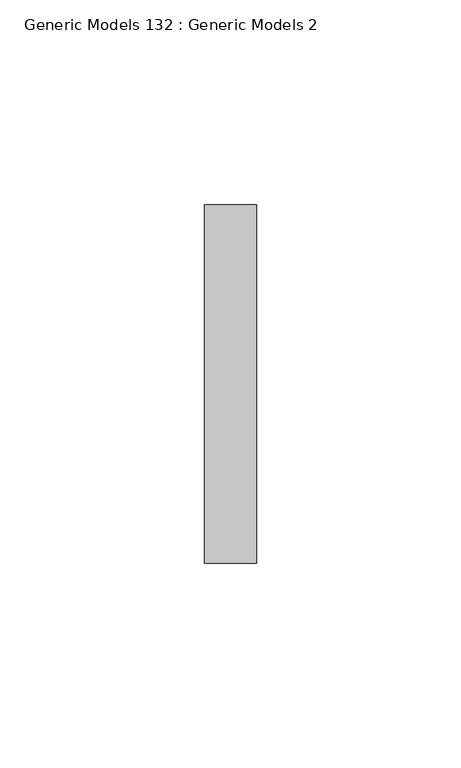
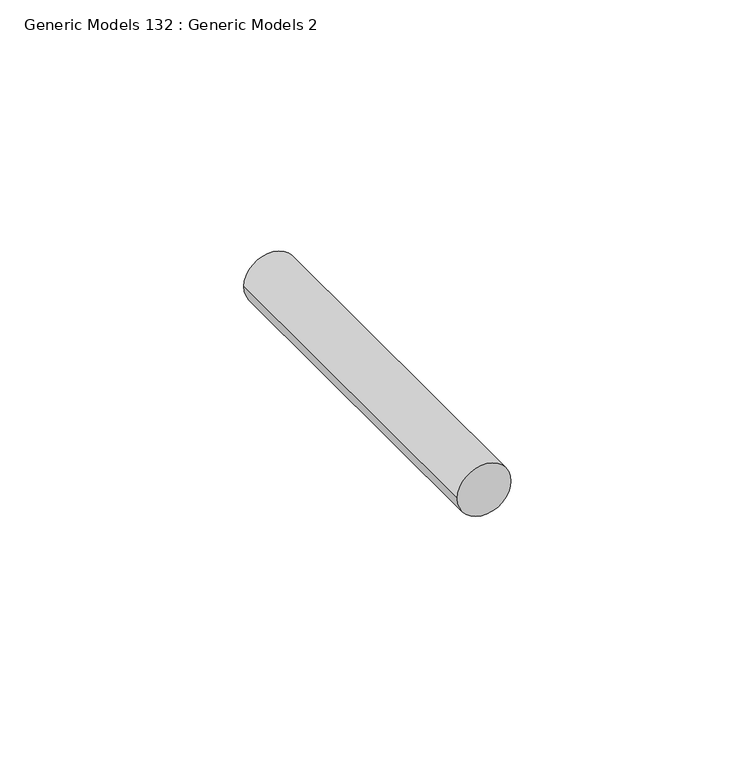
"""IFC4 building model written with IfcOpenShell, lengths in millimetres: proxy geometry, Generic Models 132 : Generic Models 2."""

from ifc_helpers import new_model, si_unit, point, frame, frame_2d, origin, place, context, project, spatial, circle_curve, trimmed, segment, composite_curve, outline, extrude, source, transform, mapped, element, save


def generic_models_132_generic_models_2_3afdd28c(model_context):
    return source(origin(), model_context, "Body", "SweptSolid", [
        extrude(outline(composite_curve([segment(trimmed(circle_curve(frame_2d((38546.4677238, 7856.3346014)), 6.35), [point((38546.4677238, 7862.6846014))], [point((38546.4677238, 7849.9846014))], False, "CARTESIAN"), True, "CONTINUOUS"), segment(trimmed(circle_curve(frame_2d((38546.4677238, 7856.3346014)), 6.35), [point((38546.4677238, 7849.9846014))], [point((38546.4677238, 7862.6846014))], False, "CARTESIAN"), True, "CONTINUOUS")], self_intersect=False)), frame((0.0, 1848.3666731, 0.0), z_axis=(0.0, 1.0, 0.0), x_axis=(0.0, 0.0, 1.0)), (0.0, 0.0, 1.0), 87.551022),
    ])


if __name__ == "__main__":
    model = new_model("IFC4")
    model_context = context("Model", 3, world=origin())
    ifc_project = project(units=[si_unit("LENGTHUNIT", "METRE", prefix="MILLI")], contexts=[model_context])
    site = spatial("IfcSite", under=ifc_project)
    building = spatial("IfcBuilding", under=site)
    placement = place(None, origin())
    generic_models_132_generic_models_2_shape = generic_models_132_generic_models_2_3afdd28c(model_context)
    element("IfcBuildingElementProxy", 1, Name="Generic Models 132 : Generic Models 2", ObjectType="Generic Models 132 : Generic Models 2", at=placement, inside=building, context=model_context, shape_type="MappedRepresentation", body=[
        mapped(generic_models_132_generic_models_2_shape, transform((0.0, 0.0, 0.0), x_axis=(1.0, 0.0, 0.0), y_axis=(0.0, 1.0, 0.0), z_axis=(0.0, 0.0, 1.0))),
    ])
    save(model, "model.ifc")

# Revit data of these elements
# Element 1 (IfcBuildingElementProxy, "Generic Models 132 : Generic Models 2")
#   Materials on its faces: "S.S. LAG BOLT - SEE STRUCT. DWGS"
# Materials
#   "S.S. LAG BOLT - SEE STRUCT. DWGS": class "Generic", colour RGB 120 120 120, transparency 0, Cost = 0
